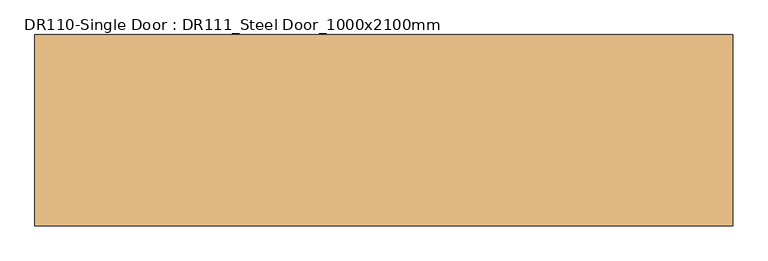
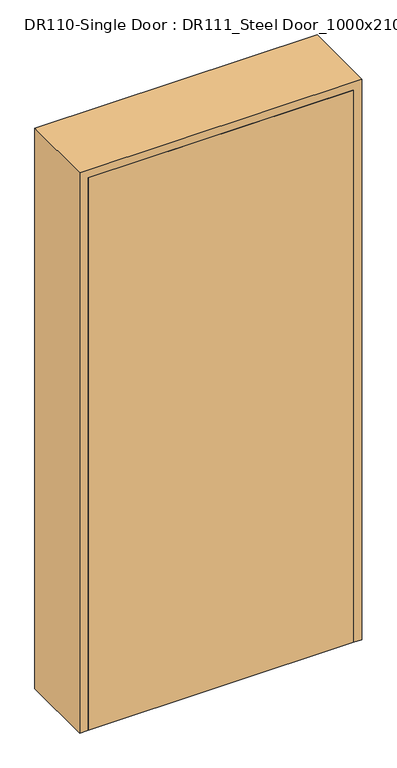
"""IFC4 building model written with IfcOpenShell, lengths in millimetres: door geometry, DR110-Single Door : DR111_Steel Door_1000x2100mm."""

import ifcopenshell
import ifcopenshell.guid

model = None  # the IFC model being written
_history = None  # IfcOwnerHistory: only IFC2X3 demands one
_inside = {}  # id of a spatial element -> (the spatial element, [elements in it])
_under = {}  # id of a project, library or spatial element -> (it, [spatial elements below it])
_declared = {}  # id of a project -> (the project, [libraries it declares])
_typed = {}  # id of a type object -> (the type object, [elements of that type])
_made_of = {}  # id of a material, layer set ... -> (it, [elements and type objects made of it])


def new_model(schema):
    """Start an empty IFC model of exactly this schema.

    Asked for "IFC4X3", IfcOpenShell would pick the latest addendum, in which some entities
    have other attributes; the version numbers below select the first issue.
    IFC2X3 requires an IfcOwnerHistory on every rooted entity: one is made here for all.
    """
    global model, _history
    if schema == "IFC4X3":
        model = ifcopenshell.file(schema_version=(4, 3, 0, 0))
    else:
        model = ifcopenshell.file(schema=schema)
    _inside.clear()
    _under.clear()
    _declared.clear()
    _typed.clear()
    _made_of.clear()
    _history = None
    if model.schema == "IFC2X3":
        org = make("IfcOrganization", Name="unknown")
        user = make(
            "IfcPersonAndOrganization",
            ThePerson=make("IfcPerson", FamilyName="unknown"),
            TheOrganization=org,
        )
        app = make(
            "IfcApplication",
            ApplicationDeveloper=org,
            Version="unknown",
            ApplicationFullName="unknown",
            ApplicationIdentifier="unknown",
        )
        _history = make(
            "IfcOwnerHistory",
            OwningUser=user,
            OwningApplication=app,
            ChangeAction="ADDED",
            CreationDate=0,
        )
    return model


def make(cls, **values):
    """One entity of the class cls with the attributes given. An attribute that is None is left unset."""
    return model.create_entity(
        cls, **{name: value for name, value in values.items() if value is not None}
    )


def rooted(cls, **values):
    """An entity with a GlobalId (a new one), such as an element, a storey or a relation."""
    return make(cls, GlobalId=ifcopenshell.guid.new(), OwnerHistory=_history, **values)


def si_unit(unit_type, name, prefix=None):
    """IfcSIUnit, for example si_unit("LENGTHUNIT", "METRE", prefix="MILLI")."""
    return make("IfcSIUnit", UnitType=unit_type, Prefix=prefix, Name=name)


def assignment(units):
    """IfcUnitAssignment: the units of a project."""
    return None if units is None else make("IfcUnitAssignment", Units=units)


def point(xyz):
    """IfcCartesianPoint."""
    return None if xyz is None else make("IfcCartesianPoint", Coordinates=xyz)


def direction(xyz):
    """IfcDirection."""
    return None if xyz is None else make("IfcDirection", DirectionRatios=xyz)


def frame(location, z_axis=None, x_axis=None):
    """IfcAxis2Placement3D, a coordinate frame: its origin and axes. An axis left out is left unset."""
    return make(
        "IfcAxis2Placement3D",
        Location=point(location),
        Axis=direction(z_axis),
        RefDirection=direction(x_axis),
    )


def origin():
    """The frame at (0, 0, 0) with its axes left unset."""
    return frame((0.0, 0.0, 0.0))


def origin_with_axes():
    """The frame at (0, 0, 0) with the z axis (0, 0, 1) and the x axis (1, 0, 0) written out."""
    return frame((0.0, 0.0, 0.0), z_axis=(0.0, 0.0, 1.0), x_axis=(1.0, 0.0, 0.0))


def place(relative_to, where):
    """IfcLocalPlacement: puts the frame where relative to a parent placement (None: the world)."""
    return make(
        "IfcLocalPlacement", PlacementRelTo=relative_to, RelativePlacement=where
    )


def context(
    kind, dimensions, precision=None, world=None, true_north=None, identifier=None
):
    """IfcGeometricRepresentationContext, for example the 3D "Model" context."""
    return make(
        "IfcGeometricRepresentationContext",
        ContextIdentifier=identifier,
        ContextType=kind,
        CoordinateSpaceDimension=dimensions,
        Precision=precision,
        WorldCoordinateSystem=world,
        TrueNorth=true_north,
    )


def project(units=None, contexts=None):
    """IfcProject with its units and contexts."""
    return rooted(
        "IfcProject",
        Name="project",
        RepresentationContexts=contexts,
        UnitsInContext=assignment(units),
    )


def spatial(cls, under=None, at=None, **own):
    """A site, building, storey or space (cls), placed at a placement, below another one or the project."""
    s = rooted(cls, ObjectPlacement=at, **own)
    if under is not None:
        _under.setdefault(under.id(), (under, []))[1].append(s)
    return s


def polyline(points):
    """IfcPolyline through the points."""
    return make("IfcPolyline", Points=[point(p) for p in points])


def outline(outer, holes=None, kind="AREA"):
    """IfcArbitraryClosedProfileDef: a profile drawn as a closed curve; with holes, ...WithVoids."""
    if holes is None:
        return make("IfcArbitraryClosedProfileDef", ProfileType=kind, OuterCurve=outer)
    return make(
        "IfcArbitraryProfileDefWithVoids",
        ProfileType=kind,
        OuterCurve=outer,
        InnerCurves=holes,
    )


def extrude(swept, where, along, depth):
    """IfcExtrudedAreaSolid: the profile swept, set in the frame where, extruded along a direction by depth."""
    return make(
        "IfcExtrudedAreaSolid",
        SweptArea=swept,
        Position=where,
        ExtrudedDirection=direction(along),
        Depth=depth,
    )


def faces_of(points, faces, orient=None, outer=None):
    """IfcFace entities. A face is a list of loops; a loop is a list of indices into points, from 0.

    orient and outer hold one flag for each loop. By default every Orientation is true, the
    first loop of a face is its IfcFaceOuterBound and the others are IfcFaceBound.
    """
    made = []
    for i, loops in enumerate(faces):
        bounds = []
        for j, loop in enumerate(loops):
            is_outer = j == 0 if outer is None else outer[i][j]
            bounds.append(
                make(
                    "IfcFaceOuterBound" if is_outer else "IfcFaceBound",
                    Bound=make("IfcPolyLoop", Polygon=[points[k] for k in loop]),
                    Orientation=True if orient is None else orient[i][j],
                )
            )
        made.append(make("IfcFace", Bounds=bounds))
    return made


def faceted_brep(points, faces, orient=None, outer=None, voids=None):
    """IfcFacetedBrep: a solid bounded by flat faces; with voids (closed shells), ...WithVoids."""
    shared = [point(p) for p in points]
    hull = make("IfcClosedShell", CfsFaces=faces_of(shared, faces, orient, outer))
    if voids is None:
        return make("IfcFacetedBrep", Outer=hull)
    return make(
        "IfcFacetedBrepWithVoids",
        Outer=hull,
        Voids=[
            make(cls, CfsFaces=faces_of(shared, fs, o, b)) for cls, fs, o, b in voids
        ],
    )


def shape(context_of_items, identifier, shape_type, items):
    """IfcShapeRepresentation: the items that make up one representation, for example the "Body"."""
    return make(
        "IfcShapeRepresentation",
        ContextOfItems=context_of_items,
        RepresentationIdentifier=identifier,
        RepresentationType=shape_type,
        Items=items,
    )


def source(mapping_origin, context_of_items, identifier, shape_type, items):
    """IfcRepresentationMap: a shape defined once, which mapped items show again and again."""
    return make(
        "IfcRepresentationMap",
        MappingOrigin=mapping_origin,
        MappedRepresentation=shape(context_of_items, identifier, shape_type, items),
    )


def transform(
    local_origin,
    x_axis=None,
    y_axis=None,
    z_axis=None,
    scale=None,
    scale2=None,
    scale3=None,
    uniform=True,
):
    """IfcCartesianTransformationOperator3D, or its non-uniform kind. x_axis, y_axis, z_axis: its Axis1, 2, 3."""
    if uniform:
        return make(
            "IfcCartesianTransformationOperator3D",
            Axis1=direction(x_axis),
            Axis2=direction(y_axis),
            LocalOrigin=point(local_origin),
            Scale=scale,
            Axis3=direction(z_axis),
        )
    return make(
        "IfcCartesianTransformationOperator3DnonUniform",
        Axis1=direction(x_axis),
        Axis2=direction(y_axis),
        LocalOrigin=point(local_origin),
        Scale=scale,
        Axis3=direction(z_axis),
        Scale2=scale2,
        Scale3=scale3,
    )


def mapped(mapping_source, mapping_target):
    """IfcMappedItem: shows the shape of a source again, moved by a transform."""
    return make(
        "IfcMappedItem", MappingSource=mapping_source, MappingTarget=mapping_target
    )


def made_of(thing, what):
    """Note that an element or type object is made of a material, layer set ...; save() writes the relation."""
    if what is not None:
        _made_of.setdefault(what.id(), (what, []))[1].append(thing)
    return thing


def element(
    cls,
    number,
    at=None,
    inside=None,
    cuts=None,
    type_object=None,
    material=None,
    context=None,
    identifier="Body",
    shape_type=None,
    held_by="IfcProductDefinitionShape",
    body=None,
    shapes=None,
    **own,
):
    """One element of the class cls, such as IfcWall. Its Tag is "e" and its number.

    at: its placement. inside: the storey or other place that contains it. cuts: it is an
    opening in that element (IfcRelVoidsElement). A single representation is given by context,
    identifier, shape_type and body (its items); several are given by shapes. held_by: the class
    of the entity that holds the representations. save() writes the other relations.
    """
    e = rooted(cls, Tag="e%d" % number, ObjectPlacement=at, **own)
    if body is not None:
        shapes = [shape(context, identifier, shape_type, body)]
    if shapes is not None:
        e.Representation = make(held_by, Representations=shapes)
    if inside is not None:
        _inside.setdefault(inside.id(), (inside, []))[1].append(e)
    if cuts is not None:
        rooted(
            "IfcRelVoidsElement", RelatingBuildingElement=cuts, RelatedOpeningElement=e
        )
    if type_object is not None:
        _typed.setdefault(type_object.id(), (type_object, []))[1].append(e)
    return made_of(e, material)


def aggregate(whole, parts):
    """IfcRelAggregates: a whole, such as a stair, and the parts it consists of."""
    return rooted("IfcRelAggregates", RelatingObject=whole, RelatedObjects=parts)


def save(model, path):
    """Write the relations noted so far, then the file.

    IfcRelAggregates (storeys below a building ...), IfcRelContainedInSpatialStructure (elements
    in a storey), IfcRelDefinesByType, IfcRelAssociatesMaterial and IfcRelDeclares: one each for
    every whole, place, type object, material and project.
    """
    for whole, parts in _under.values():
        aggregate(whole, parts)
    for where, things in _inside.values():
        rooted(
            "IfcRelContainedInSpatialStructure",
            RelatedElements=things,
            RelatingStructure=where,
        )
    for kind, things in _typed.values():
        rooted("IfcRelDefinesByType", RelatedObjects=things, RelatingType=kind)
    for what, things in _made_of.values():
        rooted("IfcRelAssociatesMaterial", RelatedObjects=things, RelatingMaterial=what)
    for by, libraries in _declared.values():
        rooted("IfcRelDeclares", RelatingContext=by, RelatedDefinitions=libraries)
    model.write(path)


def dr110_single_door_dr111_steel_door_1000x2100mm_c730d40a(model_context):
    return source(origin(), model_context, "Body", "SolidModel", [
        extrude(outline(polyline([(470.0, -137.0), (-470.0, -137.0), (-470.0, -102.0), (470.0, -102.0), (470.0, -137.0)])), origin_with_axes(), (0.0, 0.0, 1.0), 2070.0),
        faceted_brep([(470.0, -137.0, 0.0), (470.0, -102.0, 0.0), (450.0, -102.0, 0.0), (450.0, 102.0, 0.0), (470.0, 102.0, 0.0), (470.0, 137.0, 0.0), (500.0, 137.0, 0.0), (500.0, -137.0, 0.0), (500.0, -137.0, 2100.0), (-500.0, -137.0, 2100.0), (-500.0, -137.0, 0.0), (-470.0, -137.0, 0.0), (-470.0, -137.0, 2070.0), (470.0, -137.0, 2070.0), (500.0, 137.0, 2100.0), (470.0, 137.0, 2070.0), (-470.0, 137.0, 2070.0), (-470.0, 137.0, 0.0), (-500.0, 137.0, 0.0), (-500.0, 137.0, 2100.0), (470.0, 102.0, 2070.0), (450.0, 102.0, 2050.0), (-450.0, 102.0, 2050.0), (-450.0, 102.0, 0.0), (-470.0, 102.0, 0.0), (-470.0, 102.0, 2070.0), (450.0, -102.0, 2050.0), (470.0, -102.0, 2070.0), (-470.0, -102.0, 2070.0), (-470.0, -102.0, 0.0), (-450.0, -102.0, 0.0), (-450.0, -102.0, 2050.0)], [[[0, 1, 2, 3, 4, 5, 6, 7]], [[7, 8, 9, 10, 11, 12, 13, 0]], [[6, 14, 8, 7]], [[5, 15, 16, 17, 18, 19, 14, 6]], [[4, 20, 15, 5]], [[3, 21, 22, 23, 24, 25, 20, 4]], [[2, 26, 21, 3]], [[1, 27, 28, 29, 30, 31, 26, 2]], [[0, 13, 27, 1]], [[12, 11, 29, 28]], [[11, 10, 18, 17, 24, 23, 30, 29]], [[19, 18, 10, 9]], [[25, 24, 17, 16]], [[31, 30, 23, 22]], [[14, 19, 9, 8]], [[20, 25, 16, 15]], [[26, 31, 22, 21]], [[13, 12, 28, 27]]]),
    ])


if __name__ == "__main__":
    model = new_model("IFC4")
    model_context = context("Model", 3, world=origin())
    ifc_project = project(units=[si_unit("LENGTHUNIT", "METRE", prefix="MILLI")], contexts=[model_context])
    site = spatial("IfcSite", under=ifc_project)
    building = spatial("IfcBuilding", under=site)
    placement = place(None, origin())
    dr110_single_door_dr111_steel_door_1000x2100mm_shape = dr110_single_door_dr111_steel_door_1000x2100mm_c730d40a(model_context)
    element("IfcDoor", 1, ObjectType="DR110-Single Door : DR111_Steel Door_1000x2100mm", at=placement, inside=building, context=model_context, shape_type="MappedRepresentation", body=[
        mapped(dr110_single_door_dr111_steel_door_1000x2100mm_shape, transform((0.0, 0.0, 0.0), x_axis=(1.0, 0.0, 0.0), y_axis=(0.0, 1.0, 0.0), z_axis=(0.0, 0.0, 1.0))),
    ])
    save(model, "model.ifc")

# Revit data of these elements
# Type "DR110-Single Door : DR111_Steel Door_1000x2100mm"
#   Type Mark = "SD"
#   Analytic Construction = "<None>"
#   프레임 투영 외부. = 25 mm
#   프레임 투영 내부. = 25 mm
#   프레임 폭 = 75 mm
#   Height = 2100 mm
#   Width = 1000 mm
#   Define Thermal Properties by = 1
#   문 패널 = SD1 문 패널
#   문 프레임 = A04AQ098-00002_Steel Door_non FP_single
#   Function = (empty or 0)
#   Wall Closure = (empty or 0)
# Element 1 (IfcDoor, "DR110-Single Door : DR111_Steel Door_1000x2100mm")
#   Materials on its faces: "A04AQ098-00002_Steel Door_non FP_single", "SD1 문 패널"
# Materials
#   "SD1 문 패널": class "금속", colour RGB 247 247 247, transparency 0, Description = "STEEL DOOR (1000Wx2100H)"
#   "A04AQ098-00002_Steel Door_non FP_single": class "금속", colour RGB 247 247 247, transparency 0, Description = "Steel Door", W00) Work Master Code = "A04AQ098-00002", W01) Work Master_Lv1 = "Finishing Work", W02) Work Master_Lv2 = "Door & Window Work", W03) Work Master_Spec.1 = "Steel Door w/ Steel Frame", W04) Work Master_Spec.2 = "Fire Protective Rating: N/A, Single Door", W05) Work Master_Spec.3 = "w/ Hardware & Accessories", Cost = 0
